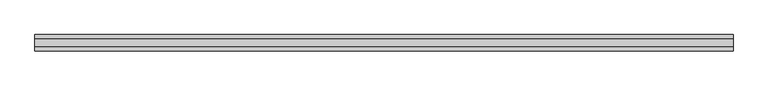
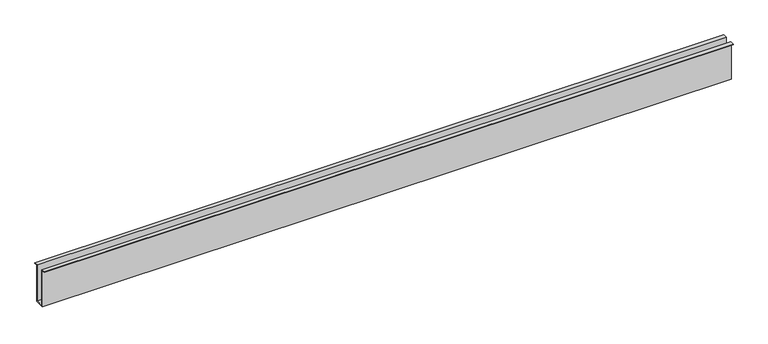
"""IFC4 building model written with IfcOpenShell, lengths in millimetres: railing geometry, ML_Perfil U de embutir3 : ML_Perfil U de embutir."""

import ifcopenshell
import ifcopenshell.guid

model = None  # the IFC model being written
_history = None  # IfcOwnerHistory: only IFC2X3 demands one
_inside = {}  # id of a spatial element -> (the spatial element, [elements in it])
_under = {}  # id of a project, library or spatial element -> (it, [spatial elements below it])
_declared = {}  # id of a project -> (the project, [libraries it declares])
_typed = {}  # id of a type object -> (the type object, [elements of that type])
_made_of = {}  # id of a material, layer set ... -> (it, [elements and type objects made of it])


def new_model(schema):
    """Start an empty IFC model of exactly this schema.

    Asked for "IFC4X3", IfcOpenShell would pick the latest addendum, in which some entities
    have other attributes; the version numbers below select the first issue.
    IFC2X3 requires an IfcOwnerHistory on every rooted entity: one is made here for all.
    """
    global model, _history
    if schema == "IFC4X3":
        model = ifcopenshell.file(schema_version=(4, 3, 0, 0))
    else:
        model = ifcopenshell.file(schema=schema)
    _inside.clear()
    _under.clear()
    _declared.clear()
    _typed.clear()
    _made_of.clear()
    _history = None
    if model.schema == "IFC2X3":
        org = make("IfcOrganization", Name="unknown")
        user = make(
            "IfcPersonAndOrganization",
            ThePerson=make("IfcPerson", FamilyName="unknown"),
            TheOrganization=org,
        )
        app = make(
            "IfcApplication",
            ApplicationDeveloper=org,
            Version="unknown",
            ApplicationFullName="unknown",
            ApplicationIdentifier="unknown",
        )
        _history = make(
            "IfcOwnerHistory",
            OwningUser=user,
            OwningApplication=app,
            ChangeAction="ADDED",
            CreationDate=0,
        )
    return model


def make(cls, **values):
    """One entity of the class cls with the attributes given. An attribute that is None is left unset."""
    return model.create_entity(
        cls, **{name: value for name, value in values.items() if value is not None}
    )


def rooted(cls, **values):
    """An entity with a GlobalId (a new one), such as an element, a storey or a relation."""
    return make(cls, GlobalId=ifcopenshell.guid.new(), OwnerHistory=_history, **values)


def si_unit(unit_type, name, prefix=None):
    """IfcSIUnit, for example si_unit("LENGTHUNIT", "METRE", prefix="MILLI")."""
    return make("IfcSIUnit", UnitType=unit_type, Prefix=prefix, Name=name)


def assignment(units):
    """IfcUnitAssignment: the units of a project."""
    return None if units is None else make("IfcUnitAssignment", Units=units)


def point(xyz):
    """IfcCartesianPoint."""
    return None if xyz is None else make("IfcCartesianPoint", Coordinates=xyz)


def direction(xyz):
    """IfcDirection."""
    return None if xyz is None else make("IfcDirection", DirectionRatios=xyz)


def frame(location, z_axis=None, x_axis=None):
    """IfcAxis2Placement3D, a coordinate frame: its origin and axes. An axis left out is left unset."""
    return make(
        "IfcAxis2Placement3D",
        Location=point(location),
        Axis=direction(z_axis),
        RefDirection=direction(x_axis),
    )


def origin():
    """The frame at (0, 0, 0) with its axes left unset."""
    return frame((0.0, 0.0, 0.0))


def place(relative_to, where):
    """IfcLocalPlacement: puts the frame where relative to a parent placement (None: the world)."""
    return make(
        "IfcLocalPlacement", PlacementRelTo=relative_to, RelativePlacement=where
    )


def context(
    kind, dimensions, precision=None, world=None, true_north=None, identifier=None
):
    """IfcGeometricRepresentationContext, for example the 3D "Model" context."""
    return make(
        "IfcGeometricRepresentationContext",
        ContextIdentifier=identifier,
        ContextType=kind,
        CoordinateSpaceDimension=dimensions,
        Precision=precision,
        WorldCoordinateSystem=world,
        TrueNorth=true_north,
    )


def project(units=None, contexts=None):
    """IfcProject with its units and contexts."""
    return rooted(
        "IfcProject",
        Name="project",
        RepresentationContexts=contexts,
        UnitsInContext=assignment(units),
    )


def spatial(cls, under=None, at=None, **own):
    """A site, building, storey or space (cls), placed at a placement, below another one or the project."""
    s = rooted(cls, ObjectPlacement=at, **own)
    if under is not None:
        _under.setdefault(under.id(), (under, []))[1].append(s)
    return s


def polyline(points):
    """IfcPolyline through the points."""
    return make("IfcPolyline", Points=[point(p) for p in points])


def outline(outer, holes=None, kind="AREA"):
    """IfcArbitraryClosedProfileDef: a profile drawn as a closed curve; with holes, ...WithVoids."""
    if holes is None:
        return make("IfcArbitraryClosedProfileDef", ProfileType=kind, OuterCurve=outer)
    return make(
        "IfcArbitraryProfileDefWithVoids",
        ProfileType=kind,
        OuterCurve=outer,
        InnerCurves=holes,
    )


def extrude(swept, where, along, depth):
    """IfcExtrudedAreaSolid: the profile swept, set in the frame where, extruded along a direction by depth."""
    return make(
        "IfcExtrudedAreaSolid",
        SweptArea=swept,
        Position=where,
        ExtrudedDirection=direction(along),
        Depth=depth,
    )


def shape(context_of_items, identifier, shape_type, items):
    """IfcShapeRepresentation: the items that make up one representation, for example the "Body"."""
    return make(
        "IfcShapeRepresentation",
        ContextOfItems=context_of_items,
        RepresentationIdentifier=identifier,
        RepresentationType=shape_type,
        Items=items,
    )


def source(mapping_origin, context_of_items, identifier, shape_type, items):
    """IfcRepresentationMap: a shape defined once, which mapped items show again and again."""
    return make(
        "IfcRepresentationMap",
        MappingOrigin=mapping_origin,
        MappedRepresentation=shape(context_of_items, identifier, shape_type, items),
    )


def transform(
    local_origin,
    x_axis=None,
    y_axis=None,
    z_axis=None,
    scale=None,
    scale2=None,
    scale3=None,
    uniform=True,
):
    """IfcCartesianTransformationOperator3D, or its non-uniform kind. x_axis, y_axis, z_axis: its Axis1, 2, 3."""
    if uniform:
        return make(
            "IfcCartesianTransformationOperator3D",
            Axis1=direction(x_axis),
            Axis2=direction(y_axis),
            LocalOrigin=point(local_origin),
            Scale=scale,
            Axis3=direction(z_axis),
        )
    return make(
        "IfcCartesianTransformationOperator3DnonUniform",
        Axis1=direction(x_axis),
        Axis2=direction(y_axis),
        LocalOrigin=point(local_origin),
        Scale=scale,
        Axis3=direction(z_axis),
        Scale2=scale2,
        Scale3=scale3,
    )


def mapped(mapping_source, mapping_target):
    """IfcMappedItem: shows the shape of a source again, moved by a transform."""
    return make(
        "IfcMappedItem", MappingSource=mapping_source, MappingTarget=mapping_target
    )


def made_of(thing, what):
    """Note that an element or type object is made of a material, layer set ...; save() writes the relation."""
    if what is not None:
        _made_of.setdefault(what.id(), (what, []))[1].append(thing)
    return thing


def element(
    cls,
    number,
    at=None,
    inside=None,
    cuts=None,
    type_object=None,
    material=None,
    context=None,
    identifier="Body",
    shape_type=None,
    held_by="IfcProductDefinitionShape",
    body=None,
    shapes=None,
    **own,
):
    """One element of the class cls, such as IfcWall. Its Tag is "e" and its number.

    at: its placement. inside: the storey or other place that contains it. cuts: it is an
    opening in that element (IfcRelVoidsElement). A single representation is given by context,
    identifier, shape_type and body (its items); several are given by shapes. held_by: the class
    of the entity that holds the representations. save() writes the other relations.
    """
    e = rooted(cls, Tag="e%d" % number, ObjectPlacement=at, **own)
    if body is not None:
        shapes = [shape(context, identifier, shape_type, body)]
    if shapes is not None:
        e.Representation = make(held_by, Representations=shapes)
    if inside is not None:
        _inside.setdefault(inside.id(), (inside, []))[1].append(e)
    if cuts is not None:
        rooted(
            "IfcRelVoidsElement", RelatingBuildingElement=cuts, RelatedOpeningElement=e
        )
    if type_object is not None:
        _typed.setdefault(type_object.id(), (type_object, []))[1].append(e)
    return made_of(e, material)


def aggregate(whole, parts):
    """IfcRelAggregates: a whole, such as a stair, and the parts it consists of."""
    return rooted("IfcRelAggregates", RelatingObject=whole, RelatedObjects=parts)


def save(model, path):
    """Write the relations noted so far, then the file.

    IfcRelAggregates (storeys below a building ...), IfcRelContainedInSpatialStructure (elements
    in a storey), IfcRelDefinesByType, IfcRelAssociatesMaterial and IfcRelDeclares: one each for
    every whole, place, type object, material and project.
    """
    for whole, parts in _under.values():
        aggregate(whole, parts)
    for where, things in _inside.values():
        rooted(
            "IfcRelContainedInSpatialStructure",
            RelatedElements=things,
            RelatingStructure=where,
        )
    for kind, things in _typed.values():
        rooted("IfcRelDefinesByType", RelatedObjects=things, RelatingType=kind)
    for what, things in _made_of.values():
        rooted("IfcRelAssociatesMaterial", RelatedObjects=things, RelatingMaterial=what)
    for by, libraries in _declared.values():
        rooted("IfcRelDeclares", RelatingContext=by, RelatedDefinitions=libraries)
    model.write(path)


def railing_81dbcb3b(model_context):
    return source(origin(), model_context, "Body", "SweptSolid", [
        extrude(outline(polyline([(1832.4523952, 3702.0), (1832.4523952, 3594.0), (1856.4523952, 3594.0), (1856.4523952, 3702.0), (1866.9523952, 3702.0), (1866.9523952, 3700.0), (1858.4523952, 3700.0), (1858.4523952, 3592.0), (1830.4523952, 3592.0), (1830.4523952, 3700.0), (1821.9523952, 3700.0), (1821.9523952, 3702.0), (1832.4523952, 3702.0)])), frame((-12226.1487231, 0.0, 0.0), z_axis=(1.0, 0.0, 0.0), x_axis=(0.0, 1.0, 0.0)), (0.0, 0.0, 1.0), 1940.0),
    ])


if __name__ == "__main__":
    model = new_model("IFC4")
    model_context = context("Model", 3, world=origin())
    ifc_project = project(units=[si_unit("LENGTHUNIT", "METRE", prefix="MILLI")], contexts=[model_context])
    site = spatial("IfcSite", under=ifc_project)
    building = spatial("IfcBuilding", under=site)
    placement = place(None, origin())
    railing_shape = railing_81dbcb3b(model_context)
    element("IfcRailing", 1, ObjectType="ML_Perfil U de embutir3 : ML_Perfil U de embutir", at=placement, inside=building, context=model_context, shape_type="MappedRepresentation", body=[
        mapped(railing_shape, transform((0.0, 0.0, 0.0), x_axis=(1.0, 0.0, 0.0), y_axis=(0.0, 1.0, 0.0), z_axis=(0.0, 0.0, 1.0))),
    ])
    save(model, "model.ifc")

# Revit data of these elements
# Type "ML_Perfil U de embutir3 : ML_Perfil U de embutir"
#   ME_Compr [instance default] = 1.94 m
#   ME_Material Perfil [instance default] = .ALUMÍNIO COM PINTURA ELETROSTÁTICA BRANCA
# Element 1 (IfcRailing, "ML_Perfil U de embutir3 : ML_Perfil U de embutir")
#   Materials on its faces: ".ALUMÍNIO COM PINTURA ELETROSTÁTICA BRANCA"
# Materials
#   ".ALUMÍNIO COM PINTURA ELETROSTÁTICA BRANCA": class "CC_METAIS", colour RGB 241 241 241, transparency 0, Cost = 0
